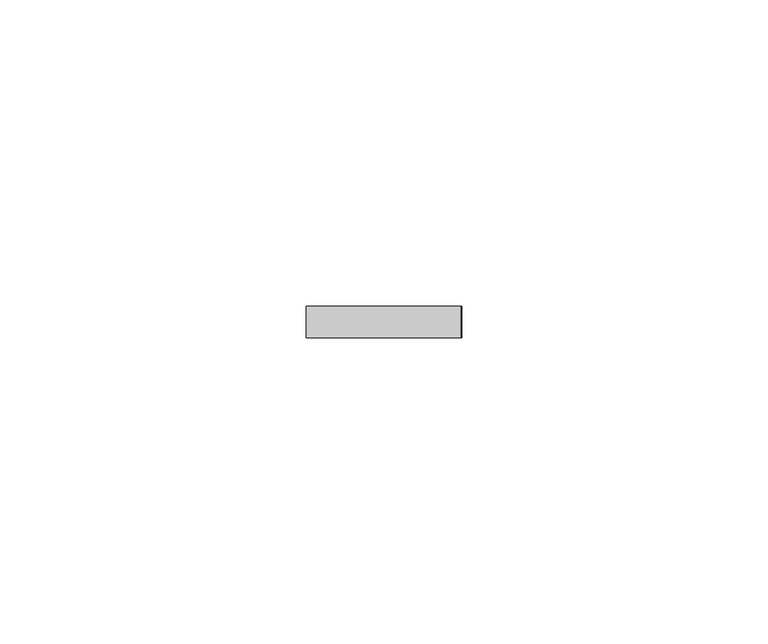
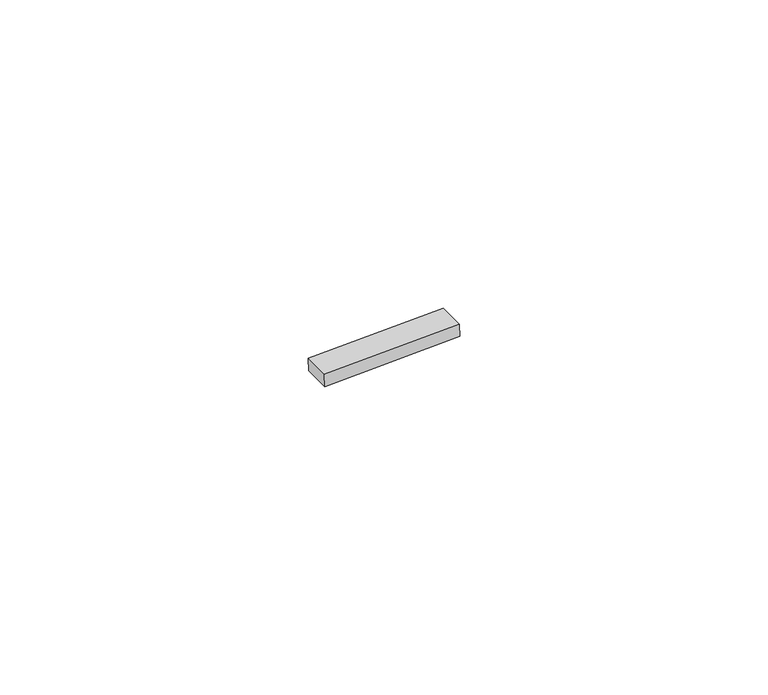
"""IFC4 building model written with IfcOpenShell, lengths in millimetres: proxy geometry, Inner panel:Inner panel:1:Inner panel:1 : Inner panel:Inner panel:300324:2:Inner panel:1:Inner panel:1 : Inner panel:Inner panel:300324:2 : Inner panel:Inner panel:1:Inner panel:1 : Inner panel:Inner panel:300324:300043:147 : Inner panel:Inner panel:1:Inner panel:1 : Inner panel:Inner panel:300324:2:Inner panel:1:Inner panel:1 : Inner panel:Inner panel:300324:2 : Inner panel:Inner panel:1:Inner panel:1 : Inner panel:Inner panel:300324:300043:308120."""

from ifc_helpers import new_model, si_unit, frame, origin, place, context, project, spatial, polyline, outline, extrude, source, transform, mapped, element, save


def generic_models_22b0906b(model_context):
    return source(origin(), model_context, "Body", "SweptSolid", [
        extrude(outline(polyline([(0.0, -25.4), (0.0, 0.0), (5.2138089, 0.0), (5.2138089, -25.4), (0.0, -25.4)])), frame((559601.0977774, -578534.9848948, 3918.0415202), z_axis=(-0.041630544712223896, 0.0, 0.9991330730923502), x_axis=(0.0, -1.0, 0.0)), (0.0, 0.0, 1.0), 2.4763745),
    ])


if __name__ == "__main__":
    model = new_model("IFC4")
    model_context = context("Model", 3, world=origin())
    ifc_project = project(units=[si_unit("LENGTHUNIT", "METRE", prefix="MILLI")], contexts=[model_context])
    site = spatial("IfcSite", under=ifc_project)
    building = spatial("IfcBuilding", under=site)
    placement = place(None, origin())
    generic_models_shape = generic_models_22b0906b(model_context)
    element("IfcBuildingElementProxy", 1, Name="Inner panel:Inner panel:1:Inner panel:1 : Inner panel:Inner panel:300324:2:Inner panel:1:Inner panel:1 : Inner panel:Inner panel:300324:2 : Inner panel:Inner panel:1:Inner panel:1 : Inner panel:Inner panel:300324:300043:147 : Inner panel:Inner panel:1:Inner panel:1 : Inner panel:Inner panel:300324:2:Inner panel:1:Inner panel:1 : Inner panel:Inner panel:300324:2 : Inner panel:Inner panel:1:Inner panel:1 : Inner panel:Inner panel:300324:300043:308120", ObjectType="Inner panel:Inner panel:1:Inner panel:1 : Inner panel:Inner panel:300324:2:Inner panel:1:Inner panel:1 : Inner panel:Inner panel:300324:2 : Inner panel:Inner panel:1:Inner panel:1 : Inner panel:Inner panel:300324:300043:147 : Inner panel:Inner panel:1:Inner panel:1 : Inner panel:Inner panel:300324:2:Inner panel:1:Inner panel:1 : Inner panel:Inner panel:300324:2 : Inner panel:Inner panel:1:Inner panel:1 : Inner panel:Inner panel:300324:300043:308120", at=placement, inside=building, context=model_context, shape_type="MappedRepresentation", body=[
        mapped(generic_models_shape, transform((0.0, 0.0, 0.0), x_axis=(1.0, 0.0, 0.0), y_axis=(0.0, 1.0, 0.0), z_axis=(0.0, 0.0, 1.0))),
    ])
    save(model, "model.ifc")

# Revit data of these elements
# Type "Inner panel:Inner panel:1:Inner panel:1 : Inner panel:Inner panel:300324:2:Inner panel:1:Inner panel:1 : Inner panel:Inner panel:300324:2 : Inner panel:Inner panel:1:Inner panel:1 : Inner panel:Inner panel:300324:300043:147 : Inner panel:Inner panel:1:Inner panel:1 : Inner panel:Inner panel:300324:2:Inner panel:1:Inner panel:1 : Inner panel:Inner panel:300324:2 : Inner panel:Inner panel:1:Inner panel:1 : Inner panel:Inner panel:300324:300043:308120"
#   NameOverride = "Inner panel:Inner panel:1:Inner panel:1 : Inner panel:Inner panel:300324:2:Inner panel:1:Inner panel:1 : Inner panel:Inner panel:300324:2 : Inner panel:Inner panel:1:Inner panel:1 : Inner panel:Inner panel:300324:300043:308120"
#   ObjectTypeOverride = "Inner panel:1:Inner panel:1 : Inner panel:Inner panel:300324:2 : Inner panel:Inner panel:1:Inner panel:1 : Inner panel:Inner panel:300324:300043"
#   Reference = "Inner panel"
#   Tag = "308120"
# Element 1 (IfcBuildingElementProxy, "Inner panel:Inner panel:1:Inner panel:1 : Inner panel:Inner panel:300324:2:Inner panel:1:Inner panel:1 : Inner panel:Inner panel:300324:2 : Inner panel:Inner panel:1:Inner panel:1 : Inner panel:Inner panel:300324:300043:147 : Inner panel:Inner panel:1:Inner panel:1 : Inner panel:Inner panel:300324:2:Inner panel:1:Inner panel:1 : Inner panel:Inner panel:300324:2 : Inner panel:Inner panel:1:Inner panel:1 : Inner panel:Inner panel:300324:300043:308120")
#   Materials on its faces: "AT CLIP - 1\" WIDE NON ABSORBENT, WEATHER-RESISTANT NEOPRENE/EPDM/SBR FOAM"
# Materials
#   "AT CLIP - 1\" WIDE NON ABSORBENT, WEATHER-RESISTANT NEOPRENE/EPDM/SBR FOAM": class "Generic", colour RGB 85 85 85, transparency 0, Cost = 0
